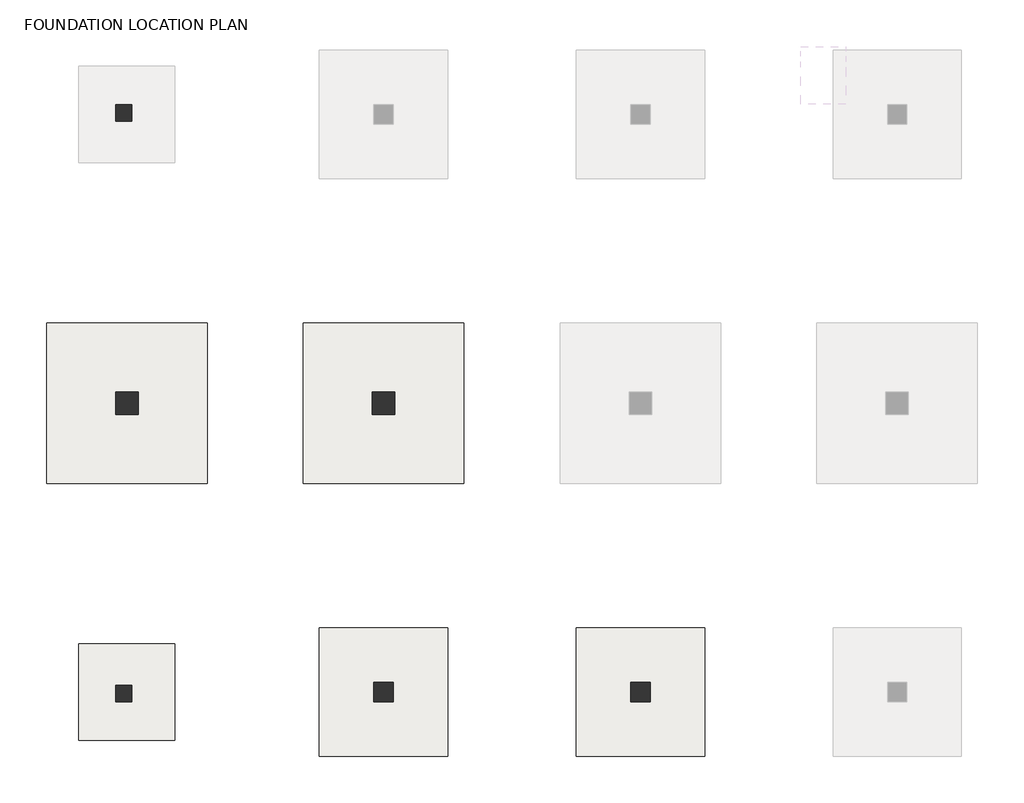
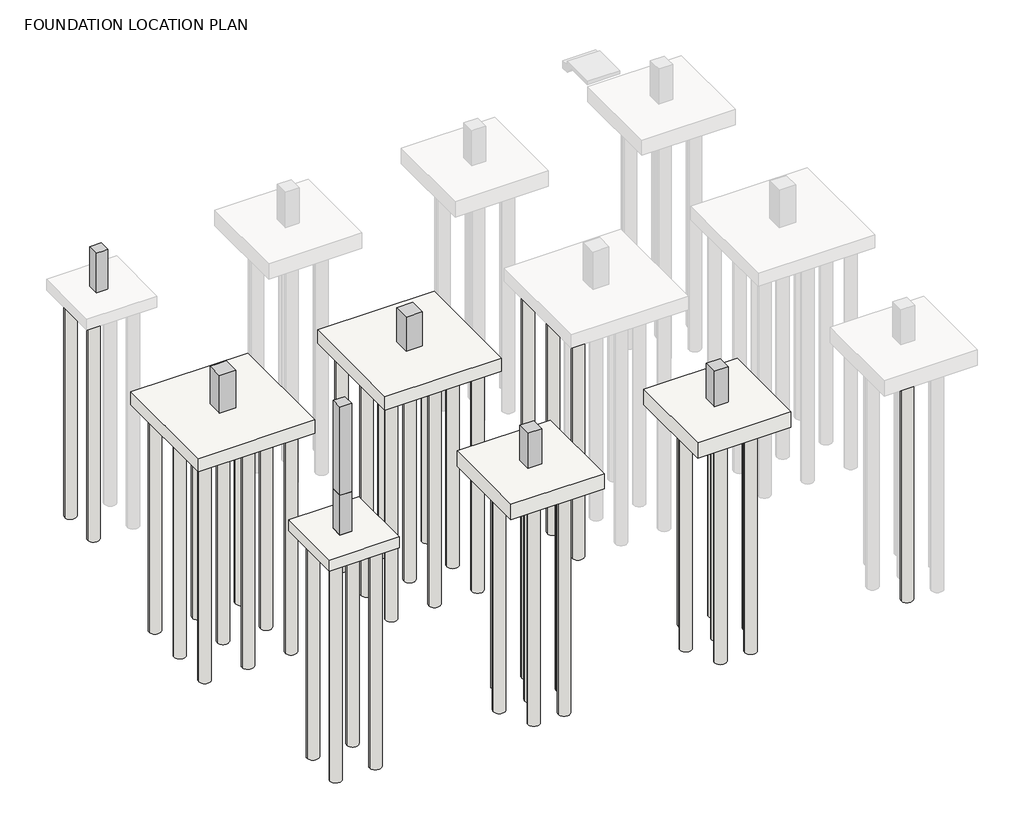
# One storey, part 1 of 3: 47 slabs, 7 columns.
"""IFC4 building model written with IfcOpenShell, lengths in millimetres."""

from ifc_helpers import new_model, si_unit, point, frame, frame_2d, origin, place, context, project, spatial, polyline, circle_curve, trimmed, segment, composite_curve, outline, extrude, faceted_brep, element, save

model = new_model("IFC4")

# Units and contexts
model_context = context("Model", 3, world=origin())
ifc_project = project(units=[si_unit("LENGTHUNIT", "METRE", prefix="MILLI")], contexts=[model_context])

# Site, building, storey
site = spatial("IfcSite", under=ifc_project)
building = spatial("IfcBuilding", under=site)
storey = spatial("IfcBuildingStorey", under=building, Name="FOUNDATION LOCATION PLAN", Elevation=-1699.994759)

# Columns
placement = place(None, origin())
element("IfcColumn", 1, ObjectType="Concrete-Rectangular-Column_R1 : CLS113_RC COLUMN_AG_C1", at=placement, inside=storey, context=model_context, shape_type="Brep", body=[
    faceted_brep([(-350.0, 21199.5208589, -1699.994759), (150.0, 21199.5208589, -1699.994759), (150.0, 20699.5208589, -1699.994759), (-350.0, 20699.5208589, -1699.994759), (150.0, 21199.5208589, -1199.994759), (-350.0, 21199.5208589, -1199.994759), (-350.0, 20699.5208589, -1199.994759), (150.0, 20699.5208589, -1199.994759)], [[[0, 1, 2, 3]], [[4, 5, 6, 7]], [[1, 0, 5, 4]], [[2, 1, 4, 7]], [[3, 2, 7, 6]], [[0, 3, 6, 5]]]),
    faceted_brep([(-350.0, 21199.5208589, 4600.005241), (150.0, 21199.5208589, 4600.005241), (150.0, 21199.5208589, 600.005241), (-99.0, 21199.5208589, 600.005241), (-350.0, 21199.5208589, 600.005241), (-350.0, 21199.5208589, 3950.005241), (-350.0, 21199.5208589, 4550.005241), (150.0, 20699.5208589, 4600.005241), (150.0, 20699.5208589, 4550.005241), (150.0, 20699.5208589, 3950.005241), (150.0, 20699.5208589, 600.005241), (150.0, 20950.5208589, 600.005241), (-350.0, 20699.5208589, 4600.005241), (-350.0, 20699.5208589, 4550.005241), (-350.0, 20699.5208589, 3950.005241), (-350.0, 20699.5208589, 600.005241)], [[[0, 1, 2, 3, 4, 5, 6]], [[1, 7, 8, 9, 10, 11, 2]], [[7, 12, 13, 14, 15, 10, 9, 8]], [[12, 0, 6, 5, 4, 15, 14, 13]], [[1, 0, 12, 7]], [[4, 3, 2, 11, 10, 15]]]),
])
element("IfcColumn", 2, ObjectType="Concrete-Rectangular-Column_R1 : CLS111_RC COLUMN_UG_C1", at=placement, inside=storey, context=model_context, shape_type="Brep", body=[
    faceted_brep([(-350.0, 21199.5208589, -1199.994759), (150.0, 21199.5208589, -1199.994759), (150.0, 20699.5208589, -1199.994759), (-350.0, 20699.5208589, -1199.994759), (-350.0, 21199.5208589, 450.005241), (-350.0, 21199.5208589, 600.005241), (150.0, 21199.5208589, 600.005241), (150.0, 21199.5208589, 450.005241), (150.0, 20699.5208589, 600.005241), (150.0, 20699.5208589, 450.005241), (-350.0, 20699.5208589, 600.005241)], [[[0, 1, 2, 3]], [[1, 0, 4, 5, 6, 7]], [[2, 1, 7, 6, 8, 9]], [[3, 2, 9, 8, 10]], [[0, 3, 10, 5, 4]], [[6, 5, 10, 8]]]),
])
element("IfcColumn", 3, ObjectType="Concrete-Rectangular-Column_R1 : CLS111_RC COLUMN_UG_C1", at=placement, inside=storey, context=model_context, shape_type="Brep", body=[
    faceted_brep([(-350.0, 39299.5208589, -1199.994759), (150.0, 39299.5208589, -1199.994759), (150.0, 38799.5208589, -1199.994759), (-350.0, 38799.5208589, -1199.994759), (-350.0, 39299.5208589, 600.005241), (150.0, 39299.5208589, 600.005241), (150.0, 38999.7368538, 600.005241), (150.0, 38799.7368538, 600.005241), (150.0, 38799.5208589, 600.005241), (150.0, 38799.5208589, 450.005241), (0.0, 38799.5208589, 600.005241), (-350.0, 38799.5208589, 600.005241), (-350.0, 38799.7368538, 600.005241)], [[[0, 1, 2, 3]], [[1, 0, 4, 5]], [[2, 1, 5, 6, 7, 8, 9]], [[3, 2, 9, 8, 10, 11]], [[0, 3, 11, 12, 4]], [[5, 4, 12, 11, 10, 8, 7, 6]]]),
])
element("IfcColumn", 4, ObjectType="Concrete-Rectangular-Column_R1 : CLS111_RC COLUMN_UG_C3", at=placement, inside=storey, context=model_context, shape_type="Brep", body=[
    faceted_brep([(-350.0, 30349.5208589, -1099.994759), (350.0, 30349.5208589, -1099.994759), (350.0, 29649.5208589, -1099.994759), (-350.0, 29649.5208589, -1099.994759), (-350.0, 30349.5208589, 600.005241), (0.0, 30349.5208589, 600.005241), (350.0, 30349.5208589, 600.005241), (350.0, 30349.5208589, 450.005241), (350.0, 29999.5208589, 600.005241), (350.0, 29649.5208589, 600.005241), (-99.0, 29649.5208589, 600.005241), (-350.0, 29649.5208589, 600.005241)], [[[0, 1, 2, 3]], [[1, 0, 4, 5, 6, 7]], [[2, 1, 7, 6, 8, 9]], [[3, 2, 9, 10, 11]], [[0, 3, 11, 4]], [[11, 10, 9, 8, 6, 5, 4]]]),
])
element("IfcColumn", 5, ObjectType="Concrete-Rectangular-Column_R1 : CLS111_RC COLUMN_UG_C3", at=placement, inside=storey, context=model_context, shape_type="SweptSolid", body=[
    extrude(outline(polyline([(7650.0, 30349.5208589), (8350.0, 30349.5208589), (8350.0, 29649.5208589), (7650.0, 29649.5208589), (7650.0, 30349.5208589)])), frame((0.0, 0.0, -1099.994759), z_axis=(0.0, 0.0, 1.0), x_axis=(1.0, 0.0, 0.0)), (0.0, 0.0, 1.0), 1550.0),
])
element("IfcColumn", 6, ObjectType="Concrete-Rectangular-Column_R1 : CLS111_RC COLUMN_UG_C2", at=placement, inside=storey, context=model_context, shape_type="Brep", body=[
    faceted_brep([(7700.0, 21299.5208589, -999.994759), (8300.0, 21299.5208589, -999.994759), (8300.0, 20699.5208589, -999.994759), (7700.0, 20699.5208589, -999.994759), (7700.0, 21299.5208589, 450.005241), (7700.0, 21299.5208589, 600.005241), (8300.0, 21299.5208589, 600.005241), (8300.0, 21299.5208589, 450.005241), (8300.0, 20999.5208589, 600.005241), (8300.0, 20699.5208589, 600.005241), (7700.0, 20699.5208589, 600.005241), (7700.0, 20999.5208589, 600.005241)], [[[0, 1, 2, 3]], [[1, 0, 4, 5, 6, 7]], [[2, 1, 7, 6, 8, 9]], [[3, 2, 9, 10]], [[0, 3, 10, 11, 5, 4]], [[6, 5, 11, 10, 9, 8]]]),
])
element("IfcColumn", 7, ObjectType="Concrete-Rectangular-Column_R1 : CLS111_RC COLUMN_UG_C2", at=placement, inside=storey, context=model_context, shape_type="Brep", body=[
    faceted_brep([(15700.0, 21299.5208589, -999.994759), (16300.0, 21299.5208589, -999.994759), (16300.0, 20699.5208589, -999.994759), (15700.0, 20699.5208589, -999.994759), (15700.0, 21299.5208589, 450.005241), (15700.0, 21299.5208589, 600.005241), (16300.0, 21299.5208589, 600.005241), (16300.0, 21299.5208589, 450.005241), (16300.0, 20999.5208589, 600.005241), (16300.0, 20699.5208589, 600.005241), (15700.0, 20699.5208589, 600.005241), (15700.0, 20999.5208589, 600.005241)], [[[0, 1, 2, 3]], [[1, 0, 4, 5, 6, 7]], [[2, 1, 7, 6, 8, 9]], [[3, 2, 9, 10]], [[0, 3, 10, 11, 5, 4]], [[6, 5, 11, 10, 9, 8]]]),
])

# Slabs
element("IfcSlab", 8, ObjectType="Footing-Rectangular_R1 : FTS301_Footing-Rectangular_3000x3000x500_F1", at=placement, inside=storey, context=model_context, shape_type="SweptSolid", body=[
    extrude(outline(polyline([(1500.0, 22499.5208589), (1500.0, 19499.5208589), (-1500.0, 19499.5208589), (-1500.0, 22499.5208589), (1500.0, 22499.5208589)])), frame((0.0, 0.0, -1699.994759), z_axis=(0.0, 0.0, 1.0), x_axis=(1.0, 0.0, 0.0)), (0.0, 0.0, 1.0), 500.0),
])
element("IfcSlab", 9, ObjectType="Footing-Rectangular_R1 : FTS301_Footing-Rectangular_4000x4000x700_F2", at=placement, inside=storey, context=model_context, shape_type="SweptSolid", body=[
    extrude(outline(polyline([(10000.0, 22999.5208589), (10000.0, 18999.5208589), (6000.0, 18999.5208589), (6000.0, 22999.5208589), (10000.0, 22999.5208589)])), frame((0.0, 0.0, -1699.994759), z_axis=(0.0, 0.0, 1.0), x_axis=(1.0, 0.0, 0.0)), (0.0, 0.0, 1.0), 700.0),
])
element("IfcSlab", 10, ObjectType="Footing-Rectangular_R1 : FTS301_Footing-Rectangular_4000x4000x700_F2", at=placement, inside=storey, context=model_context, shape_type="SweptSolid", body=[
    extrude(outline(polyline([(18000.0, 22999.5208589), (18000.0, 18999.5208589), (14000.0, 18999.5208589), (14000.0, 22999.5208589), (18000.0, 22999.5208589)])), frame((0.0, 0.0, -1699.994759), z_axis=(0.0, 0.0, 1.0), x_axis=(1.0, 0.0, 0.0)), (0.0, 0.0, 1.0), 700.0),
])
element("IfcSlab", 11, ObjectType="Footing-Rectangular_R1 : FTS301_Footing-Rectangular_5000x5000x600_F3", at=placement, inside=storey, context=model_context, shape_type="SweptSolid", body=[
    extrude(outline(polyline([(2500.0, 32499.5208589), (2500.0, 27499.5208589), (-2500.0, 27499.5208589), (-2500.0, 32499.5208589), (2500.0, 32499.5208589)])), frame((0.0, 0.0, -1699.994759), z_axis=(0.0, 0.0, 1.0), x_axis=(1.0, 0.0, 0.0)), (0.0, 0.0, 1.0), 600.0),
])
element("IfcSlab", 12, ObjectType="Footing-Rectangular_R1 : FTS301_Footing-Rectangular_5000x5000x600_F3", at=placement, inside=storey, context=model_context, shape_type="SweptSolid", body=[
    extrude(outline(polyline([(10500.0, 32499.5208589), (10500.0, 27499.5208589), (5500.0, 27499.5208589), (5500.0, 32499.5208589), (10500.0, 32499.5208589)])), frame((0.0, 0.0, -1699.994759), z_axis=(0.0, 0.0, 1.0), x_axis=(1.0, 0.0, 0.0)), (0.0, 0.0, 1.0), 600.0),
])
element("IfcSlab", 13, ObjectType="HEC_PILE : FTPS102_D500", at=placement, inside=storey, context=model_context, shape_type="SweptSolid", body=[
    extrude(outline(composite_curve([segment(trimmed(circle_curve(frame_2d((7350.0, 19649.5208589)), 250.0), [point((7600.0, 19649.5208589))], [point((7100.0, 19649.5208589))], False, "CARTESIAN"), True, "CONTINUOUS"), segment(trimmed(circle_curve(frame_2d((7350.0, 19649.5208589)), 250.0), [point((7100.0, 19649.5208589))], [point((7600.0, 19649.5208589))], False, "CARTESIAN"), True, "CONTINUOUS")], self_intersect=False)), frame((0.0, 0.0, -11749.994759), z_axis=(0.0, 0.0, 1.0), x_axis=(1.0, 0.0, 0.0)), (0.0, 0.0, 1.0), 10150.0),
])
element("IfcSlab", 14, ObjectType="HEC_PILE : FTPS102_D500", at=placement, inside=storey, context=model_context, shape_type="SweptSolid", body=[
    extrude(outline(composite_curve([segment(trimmed(circle_curve(frame_2d((8650.0, 19649.5208589)), 250.0), [point((8400.0, 19649.5208589))], [point((8900.0, 19649.5208589))], False, "CARTESIAN"), True, "CONTINUOUS"), segment(trimmed(circle_curve(frame_2d((8650.0, 19649.5208589)), 250.0), [point((8900.0, 19649.5208589))], [point((8400.0, 19649.5208589))], False, "CARTESIAN"), True, "CONTINUOUS")], self_intersect=False)), frame((0.0, 0.0, -11749.994759), z_axis=(0.0, 0.0, 1.0), x_axis=(1.0, 0.0, 0.0)), (0.0, 0.0, 1.0), 10150.0),
])
element("IfcSlab", 15, ObjectType="HEC_PILE : FTPS102_D500", at=placement, inside=storey, context=model_context, shape_type="SweptSolid", body=[
    extrude(outline(composite_curve([segment(trimmed(circle_curve(frame_2d((6650.0, 20999.5208589)), 250.0), [point((6900.0, 20999.5208589))], [point((6400.0, 20999.5208589))], False, "CARTESIAN"), True, "CONTINUOUS"), segment(trimmed(circle_curve(frame_2d((6650.0, 20999.5208589)), 250.0), [point((6400.0, 20999.5208589))], [point((6900.0, 20999.5208589))], False, "CARTESIAN"), True, "CONTINUOUS")], self_intersect=False)), frame((0.0, 0.0, -11749.994759), z_axis=(0.0, 0.0, 1.0), x_axis=(1.0, 0.0, 0.0)), (0.0, 0.0, 1.0), 10150.0),
])
element("IfcSlab", 16, ObjectType="HEC_PILE : FTPS102_D500", at=placement, inside=storey, context=model_context, shape_type="SweptSolid", body=[
    extrude(outline(composite_curve([segment(trimmed(circle_curve(frame_2d((8000.0, 20999.5208589)), 250.0), [point((8250.0, 20999.5208589))], [point((7750.0, 20999.5208589))], False, "CARTESIAN"), True, "CONTINUOUS"), segment(trimmed(circle_curve(frame_2d((8000.0, 20999.5208589)), 250.0), [point((7750.0, 20999.5208589))], [point((8250.0, 20999.5208589))], False, "CARTESIAN"), True, "CONTINUOUS")], self_intersect=False)), frame((0.0, 0.0, -11749.994759), z_axis=(0.0, 0.0, 1.0), x_axis=(1.0, 0.0, 0.0)), (0.0, 0.0, 1.0), 10150.0),
])
element("IfcSlab", 17, ObjectType="HEC_PILE : FTPS102_D500", at=placement, inside=storey, context=model_context, shape_type="SweptSolid", body=[
    extrude(outline(composite_curve([segment(trimmed(circle_curve(frame_2d((9350.0, 20999.5208589)), 250.0), [point((9100.0, 20999.5208589))], [point((9600.0, 20999.5208589))], False, "CARTESIAN"), True, "CONTINUOUS"), segment(trimmed(circle_curve(frame_2d((9350.0, 20999.5208589)), 250.0), [point((9600.0, 20999.5208589))], [point((9100.0, 20999.5208589))], False, "CARTESIAN"), True, "CONTINUOUS")], self_intersect=False)), frame((0.0, 0.0, -11749.994759), z_axis=(0.0, 0.0, 1.0), x_axis=(1.0, 0.0, 0.0)), (0.0, 0.0, 1.0), 10150.0),
])
element("IfcSlab", 18, ObjectType="HEC_PILE : FTPS102_D500", at=placement, inside=storey, context=model_context, shape_type="SweptSolid", body=[
    extrude(outline(composite_curve([segment(trimmed(circle_curve(frame_2d((7350.0, 22349.5208589)), 250.0), [point((7600.0, 22349.5208589))], [point((7100.0, 22349.5208589))], False, "CARTESIAN"), True, "CONTINUOUS"), segment(trimmed(circle_curve(frame_2d((7350.0, 22349.5208589)), 250.0), [point((7100.0, 22349.5208589))], [point((7600.0, 22349.5208589))], False, "CARTESIAN"), True, "CONTINUOUS")], self_intersect=False)), frame((0.0, 0.0, -11749.994759), z_axis=(0.0, 0.0, 1.0), x_axis=(1.0, 0.0, 0.0)), (0.0, 0.0, 1.0), 10150.0),
])
element("IfcSlab", 19, ObjectType="HEC_PILE : FTPS102_D500", at=placement, inside=storey, context=model_context, shape_type="SweptSolid", body=[
    extrude(outline(composite_curve([segment(trimmed(circle_curve(frame_2d((8650.0, 22349.5208589)), 250.0), [point((8400.0, 22349.5208589))], [point((8900.0, 22349.5208589))], False, "CARTESIAN"), True, "CONTINUOUS"), segment(trimmed(circle_curve(frame_2d((8650.0, 22349.5208589)), 250.0), [point((8900.0, 22349.5208589))], [point((8400.0, 22349.5208589))], False, "CARTESIAN"), True, "CONTINUOUS")], self_intersect=False)), frame((0.0, 0.0, -11749.994759), z_axis=(0.0, 0.0, 1.0), x_axis=(1.0, 0.0, 0.0)), (0.0, 0.0, 1.0), 10150.0),
])
element("IfcSlab", 20, ObjectType="HEC_PILE : FTPS102_D500", at=placement, inside=storey, context=model_context, shape_type="SweptSolid", body=[
    extrude(outline(composite_curve([segment(trimmed(circle_curve(frame_2d((-850.0, 39849.5208589)), 250.0), [point((-600.0, 39849.5208589))], [point((-1100.0, 39849.5208589))], False, "CARTESIAN"), True, "CONTINUOUS"), segment(trimmed(circle_curve(frame_2d((-850.0, 39849.5208589)), 250.0), [point((-1100.0, 39849.5208589))], [point((-600.0, 39849.5208589))], False, "CARTESIAN"), True, "CONTINUOUS")], self_intersect=False)), frame((0.0, 0.0, -11749.994759), z_axis=(0.0, 0.0, 1.0), x_axis=(1.0, 0.0, 0.0)), (0.0, 0.0, 1.0), 10150.0),
])
element("IfcSlab", 21, ObjectType="HEC_PILE : FTPS102_D500", at=placement, inside=storey, context=model_context, shape_type="SweptSolid", body=[
    extrude(outline(composite_curve([segment(trimmed(circle_curve(frame_2d((-850.0, 21849.5208589)), 250.0), [point((-600.0, 21849.5208589))], [point((-1100.0, 21849.5208589))], False, "CARTESIAN"), True, "CONTINUOUS"), segment(trimmed(circle_curve(frame_2d((-850.0, 21849.5208589)), 250.0), [point((-1100.0, 21849.5208589))], [point((-600.0, 21849.5208589))], False, "CARTESIAN"), True, "CONTINUOUS")], self_intersect=False)), frame((0.0, 0.0, -11749.994759), z_axis=(0.0, 0.0, 1.0), x_axis=(1.0, 0.0, 0.0)), (0.0, 0.0, 1.0), 10150.0),
])
element("IfcSlab", 22, ObjectType="HEC_PILE : FTPS102_D500", at=placement, inside=storey, context=model_context, shape_type="SweptSolid", body=[
    extrude(outline(composite_curve([segment(trimmed(circle_curve(frame_2d((850.0, 21849.5208589)), 250.0), [point((600.0, 21849.5208589))], [point((1100.0, 21849.5208589))], False, "CARTESIAN"), True, "CONTINUOUS"), segment(trimmed(circle_curve(frame_2d((850.0, 21849.5208589)), 250.0), [point((1100.0, 21849.5208589))], [point((600.0, 21849.5208589))], False, "CARTESIAN"), True, "CONTINUOUS")], self_intersect=False)), frame((0.0, 0.0, -11749.994759), z_axis=(0.0, 0.0, 1.0), x_axis=(1.0, 0.0, 0.0)), (0.0, 0.0, 1.0), 10150.0),
])
element("IfcSlab", 23, ObjectType="HEC_PILE : FTPS102_D500", at=placement, inside=storey, context=model_context, shape_type="SweptSolid", body=[
    extrude(outline(composite_curve([segment(trimmed(circle_curve(frame_2d((-850.0, 20149.5208589)), 250.0), [point((-600.0, 20149.5208589))], [point((-1100.0, 20149.5208589))], False, "CARTESIAN"), True, "CONTINUOUS"), segment(trimmed(circle_curve(frame_2d((-850.0, 20149.5208589)), 250.0), [point((-1100.0, 20149.5208589))], [point((-600.0, 20149.5208589))], False, "CARTESIAN"), True, "CONTINUOUS")], self_intersect=False)), frame((0.0, 0.0, -11749.994759), z_axis=(0.0, 0.0, 1.0), x_axis=(1.0, 0.0, 0.0)), (0.0, 0.0, 1.0), 10150.0),
])
element("IfcSlab", 24, ObjectType="HEC_PILE : FTPS102_D500", at=placement, inside=storey, context=model_context, shape_type="SweptSolid", body=[
    extrude(outline(composite_curve([segment(trimmed(circle_curve(frame_2d((850.0, 20149.5208589)), 250.0), [point((600.0, 20149.5208589))], [point((1100.0, 20149.5208589))], False, "CARTESIAN"), True, "CONTINUOUS"), segment(trimmed(circle_curve(frame_2d((850.0, 20149.5208589)), 250.0), [point((1100.0, 20149.5208589))], [point((600.0, 20149.5208589))], False, "CARTESIAN"), True, "CONTINUOUS")], self_intersect=False)), frame((0.0, 0.0, -11749.994759), z_axis=(0.0, 0.0, 1.0), x_axis=(1.0, 0.0, 0.0)), (0.0, 0.0, 1.0), 10150.0),
])
element("IfcSlab", 25, ObjectType="HEC_PILE : FTPS102_D500", at=placement, inside=storey, context=model_context, shape_type="SweptSolid", body=[
    extrude(outline(composite_curve([segment(trimmed(circle_curve(frame_2d((15350.0, 19649.5208589)), 250.0), [point((15600.0, 19649.5208589))], [point((15100.0, 19649.5208589))], False, "CARTESIAN"), True, "CONTINUOUS"), segment(trimmed(circle_curve(frame_2d((15350.0, 19649.5208589)), 250.0), [point((15100.0, 19649.5208589))], [point((15600.0, 19649.5208589))], False, "CARTESIAN"), True, "CONTINUOUS")], self_intersect=False)), frame((0.0, 0.0, -11749.994759), z_axis=(0.0, 0.0, 1.0), x_axis=(1.0, 0.0, 0.0)), (0.0, 0.0, 1.0), 10150.0),
])
element("IfcSlab", 26, ObjectType="HEC_PILE : FTPS102_D500", at=placement, inside=storey, context=model_context, shape_type="SweptSolid", body=[
    extrude(outline(composite_curve([segment(trimmed(circle_curve(frame_2d((16650.0, 19649.5208589)), 250.0), [point((16400.0, 19649.5208589))], [point((16900.0, 19649.5208589))], False, "CARTESIAN"), True, "CONTINUOUS"), segment(trimmed(circle_curve(frame_2d((16650.0, 19649.5208589)), 250.0), [point((16900.0, 19649.5208589))], [point((16400.0, 19649.5208589))], False, "CARTESIAN"), True, "CONTINUOUS")], self_intersect=False)), frame((0.0, 0.0, -11749.994759), z_axis=(0.0, 0.0, 1.0), x_axis=(1.0, 0.0, 0.0)), (0.0, 0.0, 1.0), 10150.0),
])
element("IfcSlab", 27, ObjectType="HEC_PILE : FTPS102_D500", at=placement, inside=storey, context=model_context, shape_type="SweptSolid", body=[
    extrude(outline(composite_curve([segment(trimmed(circle_curve(frame_2d((14650.0, 20999.5208589)), 250.0), [point((14900.0, 20999.5208589))], [point((14400.0, 20999.5208589))], False, "CARTESIAN"), True, "CONTINUOUS"), segment(trimmed(circle_curve(frame_2d((14650.0, 20999.5208589)), 250.0), [point((14400.0, 20999.5208589))], [point((14900.0, 20999.5208589))], False, "CARTESIAN"), True, "CONTINUOUS")], self_intersect=False)), frame((0.0, 0.0, -11749.994759), z_axis=(0.0, 0.0, 1.0), x_axis=(1.0, 0.0, 0.0)), (0.0, 0.0, 1.0), 10150.0),
])
element("IfcSlab", 28, ObjectType="HEC_PILE : FTPS102_D500", at=placement, inside=storey, context=model_context, shape_type="SweptSolid", body=[
    extrude(outline(composite_curve([segment(trimmed(circle_curve(frame_2d((16000.0, 20999.5208589)), 250.0), [point((16250.0, 20999.5208589))], [point((15750.0, 20999.5208589))], False, "CARTESIAN"), True, "CONTINUOUS"), segment(trimmed(circle_curve(frame_2d((16000.0, 20999.5208589)), 250.0), [point((15750.0, 20999.5208589))], [point((16250.0, 20999.5208589))], False, "CARTESIAN"), True, "CONTINUOUS")], self_intersect=False)), frame((0.0, 0.0, -11749.994759), z_axis=(0.0, 0.0, 1.0), x_axis=(1.0, 0.0, 0.0)), (0.0, 0.0, 1.0), 10150.0),
])
element("IfcSlab", 29, ObjectType="HEC_PILE : FTPS102_D500", at=placement, inside=storey, context=model_context, shape_type="SweptSolid", body=[
    extrude(outline(composite_curve([segment(trimmed(circle_curve(frame_2d((17350.0, 20999.5208589)), 250.0), [point((17100.0, 20999.5208589))], [point((17600.0, 20999.5208589))], False, "CARTESIAN"), True, "CONTINUOUS"), segment(trimmed(circle_curve(frame_2d((17350.0, 20999.5208589)), 250.0), [point((17600.0, 20999.5208589))], [point((17100.0, 20999.5208589))], False, "CARTESIAN"), True, "CONTINUOUS")], self_intersect=False)), frame((0.0, 0.0, -11749.994759), z_axis=(0.0, 0.0, 1.0), x_axis=(1.0, 0.0, 0.0)), (0.0, 0.0, 1.0), 10150.0),
])
element("IfcSlab", 30, ObjectType="HEC_PILE : FTPS102_D500", at=placement, inside=storey, context=model_context, shape_type="SweptSolid", body=[
    extrude(outline(composite_curve([segment(trimmed(circle_curve(frame_2d((15350.0, 22349.5208589)), 250.0), [point((15600.0, 22349.5208589))], [point((15100.0, 22349.5208589))], False, "CARTESIAN"), True, "CONTINUOUS"), segment(trimmed(circle_curve(frame_2d((15350.0, 22349.5208589)), 250.0), [point((15100.0, 22349.5208589))], [point((15600.0, 22349.5208589))], False, "CARTESIAN"), True, "CONTINUOUS")], self_intersect=False)), frame((0.0, 0.0, -11749.994759), z_axis=(0.0, 0.0, 1.0), x_axis=(1.0, 0.0, 0.0)), (0.0, 0.0, 1.0), 10150.0),
])
element("IfcSlab", 31, ObjectType="HEC_PILE : FTPS102_D500", at=placement, inside=storey, context=model_context, shape_type="SweptSolid", body=[
    extrude(outline(composite_curve([segment(trimmed(circle_curve(frame_2d((16650.0, 22349.5208589)), 250.0), [point((16400.0, 22349.5208589))], [point((16900.0, 22349.5208589))], False, "CARTESIAN"), True, "CONTINUOUS"), segment(trimmed(circle_curve(frame_2d((16650.0, 22349.5208589)), 250.0), [point((16900.0, 22349.5208589))], [point((16400.0, 22349.5208589))], False, "CARTESIAN"), True, "CONTINUOUS")], self_intersect=False)), frame((0.0, 0.0, -11749.994759), z_axis=(0.0, 0.0, 1.0), x_axis=(1.0, 0.0, 0.0)), (0.0, 0.0, 1.0), 10150.0),
])
element("IfcSlab", 32, ObjectType="HEC_PILE : FTPS102_D500", at=placement, inside=storey, context=model_context, shape_type="SweptSolid", body=[
    extrude(outline(composite_curve([segment(trimmed(circle_curve(frame_2d((23350.0, 19649.5208589)), 250.0), [point((23600.0, 19649.5208589))], [point((23100.0, 19649.5208589))], False, "CARTESIAN"), True, "CONTINUOUS"), segment(trimmed(circle_curve(frame_2d((23350.0, 19649.5208589)), 250.0), [point((23100.0, 19649.5208589))], [point((23600.0, 19649.5208589))], False, "CARTESIAN"), True, "CONTINUOUS")], self_intersect=False)), frame((0.0, 0.0, -11749.994759), z_axis=(0.0, 0.0, 1.0), x_axis=(1.0, 0.0, 0.0)), (0.0, 0.0, 1.0), 10150.0),
])
element("IfcSlab", 33, ObjectType="HEC_PILE : FTPS102_D500", at=placement, inside=storey, context=model_context, shape_type="SweptSolid", body=[
    extrude(outline(composite_curve([segment(trimmed(circle_curve(frame_2d((-1850.0, 29999.5208589)), 250.0), [point((-1600.0, 29999.5208589))], [point((-2100.0, 29999.5208589))], False, "CARTESIAN"), True, "CONTINUOUS"), segment(trimmed(circle_curve(frame_2d((-1850.0, 29999.5208589)), 250.0), [point((-2100.0, 29999.5208589))], [point((-1600.0, 29999.5208589))], False, "CARTESIAN"), True, "CONTINUOUS")], self_intersect=False)), frame((0.0, 0.0, -11749.994759), z_axis=(0.0, 0.0, 1.0), x_axis=(1.0, 0.0, 0.0)), (0.0, 0.0, 1.0), 10150.0),
])
element("IfcSlab", 34, ObjectType="HEC_PILE : FTPS102_D500", at=placement, inside=storey, context=model_context, shape_type="SweptSolid", body=[
    extrude(outline(composite_curve([segment(trimmed(circle_curve(frame_2d((1850.0, 29999.5208589)), 250.0), [point((1600.0, 29999.5208589))], [point((2100.0, 29999.5208589))], False, "CARTESIAN"), True, "CONTINUOUS"), segment(trimmed(circle_curve(frame_2d((1850.0, 29999.5208589)), 250.0), [point((2100.0, 29999.5208589))], [point((1600.0, 29999.5208589))], False, "CARTESIAN"), True, "CONTINUOUS")], self_intersect=False)), frame((0.0, 0.0, -11749.994759), z_axis=(0.0, 0.0, 1.0), x_axis=(1.0, 0.0, 0.0)), (0.0, 0.0, 1.0), 10150.0),
])
element("IfcSlab", 35, ObjectType="HEC_PILE : FTPS102_D500", at=placement, inside=storey, context=model_context, shape_type="SweptSolid", body=[
    extrude(outline(composite_curve([segment(trimmed(circle_curve(frame_2d((0.0, 29999.5208589)), 250.0), [point((-250.0, 29999.5208589))], [point((250.0, 29999.5208589))], False, "CARTESIAN"), True, "CONTINUOUS"), segment(trimmed(circle_curve(frame_2d((0.0, 29999.5208589)), 250.0), [point((250.0, 29999.5208589))], [point((-250.0, 29999.5208589))], False, "CARTESIAN"), True, "CONTINUOUS")], self_intersect=False)), frame((0.0, 0.0, -11749.994759), z_axis=(0.0, 0.0, 1.0), x_axis=(1.0, 0.0, 0.0)), (0.0, 0.0, 1.0), 10150.0),
])
element("IfcSlab", 36, ObjectType="HEC_PILE : FTPS102_D500", at=placement, inside=storey, context=model_context, shape_type="SweptSolid", body=[
    extrude(outline(composite_curve([segment(trimmed(circle_curve(frame_2d((-1850.0, 31849.5208589)), 250.0), [point((-1600.0, 31849.5208589))], [point((-2100.0, 31849.5208589))], False, "CARTESIAN"), True, "CONTINUOUS"), segment(trimmed(circle_curve(frame_2d((-1850.0, 31849.5208589)), 250.0), [point((-2100.0, 31849.5208589))], [point((-1600.0, 31849.5208589))], False, "CARTESIAN"), True, "CONTINUOUS")], self_intersect=False)), frame((0.0, 0.0, -11749.994759), z_axis=(0.0, 0.0, 1.0), x_axis=(1.0, 0.0, 0.0)), (0.0, 0.0, 1.0), 10150.0),
])
element("IfcSlab", 37, ObjectType="HEC_PILE : FTPS102_D500", at=placement, inside=storey, context=model_context, shape_type="SweptSolid", body=[
    extrude(outline(composite_curve([segment(trimmed(circle_curve(frame_2d((1850.0, 31849.5208589)), 250.0), [point((1600.0, 31849.5208589))], [point((2100.0, 31849.5208589))], False, "CARTESIAN"), True, "CONTINUOUS"), segment(trimmed(circle_curve(frame_2d((1850.0, 31849.5208589)), 250.0), [point((2100.0, 31849.5208589))], [point((1600.0, 31849.5208589))], False, "CARTESIAN"), True, "CONTINUOUS")], self_intersect=False)), frame((0.0, 0.0, -11749.994759), z_axis=(0.0, 0.0, 1.0), x_axis=(1.0, 0.0, 0.0)), (0.0, 0.0, 1.0), 10150.0),
])
element("IfcSlab", 38, ObjectType="HEC_PILE : FTPS102_D500", at=placement, inside=storey, context=model_context, shape_type="SweptSolid", body=[
    extrude(outline(composite_curve([segment(trimmed(circle_curve(frame_2d((0.0, 31849.5208589)), 250.0), [point((-250.0, 31849.5208589))], [point((250.0, 31849.5208589))], False, "CARTESIAN"), True, "CONTINUOUS"), segment(trimmed(circle_curve(frame_2d((0.0, 31849.5208589)), 250.0), [point((250.0, 31849.5208589))], [point((-250.0, 31849.5208589))], False, "CARTESIAN"), True, "CONTINUOUS")], self_intersect=False)), frame((0.0, 0.0, -11749.994759), z_axis=(0.0, 0.0, 1.0), x_axis=(1.0, 0.0, 0.0)), (0.0, 0.0, 1.0), 10150.0),
])
element("IfcSlab", 39, ObjectType="HEC_PILE : FTPS102_D500", at=placement, inside=storey, context=model_context, shape_type="SweptSolid", body=[
    extrude(outline(composite_curve([segment(trimmed(circle_curve(frame_2d((-1850.0, 28149.5208589)), 250.0), [point((-1600.0, 28149.5208589))], [point((-2100.0, 28149.5208589))], False, "CARTESIAN"), True, "CONTINUOUS"), segment(trimmed(circle_curve(frame_2d((-1850.0, 28149.5208589)), 250.0), [point((-2100.0, 28149.5208589))], [point((-1600.0, 28149.5208589))], False, "CARTESIAN"), True, "CONTINUOUS")], self_intersect=False)), frame((0.0, 0.0, -11749.994759), z_axis=(0.0, 0.0, 1.0), x_axis=(1.0, 0.0, 0.0)), (0.0, 0.0, 1.0), 10150.0),
])
element("IfcSlab", 40, ObjectType="HEC_PILE : FTPS102_D500", at=placement, inside=storey, context=model_context, shape_type="SweptSolid", body=[
    extrude(outline(composite_curve([segment(trimmed(circle_curve(frame_2d((1850.0, 28149.5208589)), 250.0), [point((1600.0, 28149.5208589))], [point((2100.0, 28149.5208589))], False, "CARTESIAN"), True, "CONTINUOUS"), segment(trimmed(circle_curve(frame_2d((1850.0, 28149.5208589)), 250.0), [point((2100.0, 28149.5208589))], [point((1600.0, 28149.5208589))], False, "CARTESIAN"), True, "CONTINUOUS")], self_intersect=False)), frame((0.0, 0.0, -11749.994759), z_axis=(0.0, 0.0, 1.0), x_axis=(1.0, 0.0, 0.0)), (0.0, 0.0, 1.0), 10150.0),
])
element("IfcSlab", 41, ObjectType="HEC_PILE : FTPS102_D500", at=placement, inside=storey, context=model_context, shape_type="SweptSolid", body=[
    extrude(outline(composite_curve([segment(trimmed(circle_curve(frame_2d((0.0, 28149.5208589)), 250.0), [point((-250.0, 28149.5208589))], [point((250.0, 28149.5208589))], False, "CARTESIAN"), True, "CONTINUOUS"), segment(trimmed(circle_curve(frame_2d((0.0, 28149.5208589)), 250.0), [point((250.0, 28149.5208589))], [point((-250.0, 28149.5208589))], False, "CARTESIAN"), True, "CONTINUOUS")], self_intersect=False)), frame((0.0, 0.0, -11749.994759), z_axis=(0.0, 0.0, 1.0), x_axis=(1.0, 0.0, 0.0)), (0.0, 0.0, 1.0), 10150.0),
])
element("IfcSlab", 42, ObjectType="HEC_PILE : FTPS102_D500", at=placement, inside=storey, context=model_context, shape_type="SweptSolid", body=[
    extrude(outline(composite_curve([segment(trimmed(circle_curve(frame_2d((6150.0, 29999.5208589)), 250.0), [point((6400.0, 29999.5208589))], [point((5900.0, 29999.5208589))], False, "CARTESIAN"), True, "CONTINUOUS"), segment(trimmed(circle_curve(frame_2d((6150.0, 29999.5208589)), 250.0), [point((5900.0, 29999.5208589))], [point((6400.0, 29999.5208589))], False, "CARTESIAN"), True, "CONTINUOUS")], self_intersect=False)), frame((0.0, 0.0, -11749.994759), z_axis=(0.0, 0.0, 1.0), x_axis=(1.0, 0.0, 0.0)), (0.0, 0.0, 1.0), 10150.0),
])
element("IfcSlab", 43, ObjectType="HEC_PILE : FTPS102_D500", at=placement, inside=storey, context=model_context, shape_type="SweptSolid", body=[
    extrude(outline(composite_curve([segment(trimmed(circle_curve(frame_2d((9850.0, 29999.5208589)), 250.0), [point((9600.0, 29999.5208589))], [point((10100.0, 29999.5208589))], False, "CARTESIAN"), True, "CONTINUOUS"), segment(trimmed(circle_curve(frame_2d((9850.0, 29999.5208589)), 250.0), [point((10100.0, 29999.5208589))], [point((9600.0, 29999.5208589))], False, "CARTESIAN"), True, "CONTINUOUS")], self_intersect=False)), frame((0.0, 0.0, -11749.994759), z_axis=(0.0, 0.0, 1.0), x_axis=(1.0, 0.0, 0.0)), (0.0, 0.0, 1.0), 10150.0),
])
element("IfcSlab", 44, ObjectType="HEC_PILE : FTPS102_D500", at=placement, inside=storey, context=model_context, shape_type="SweptSolid", body=[
    extrude(outline(composite_curve([segment(trimmed(circle_curve(frame_2d((8000.0, 29999.5208589)), 250.0), [point((7750.0, 29999.5208589))], [point((8250.0, 29999.5208589))], False, "CARTESIAN"), True, "CONTINUOUS"), segment(trimmed(circle_curve(frame_2d((8000.0, 29999.5208589)), 250.0), [point((8250.0, 29999.5208589))], [point((7750.0, 29999.5208589))], False, "CARTESIAN"), True, "CONTINUOUS")], self_intersect=False)), frame((0.0, 0.0, -11749.994759), z_axis=(0.0, 0.0, 1.0), x_axis=(1.0, 0.0, 0.0)), (0.0, 0.0, 1.0), 10150.0),
])
element("IfcSlab", 45, ObjectType="HEC_PILE : FTPS102_D500", at=placement, inside=storey, context=model_context, shape_type="SweptSolid", body=[
    extrude(outline(composite_curve([segment(trimmed(circle_curve(frame_2d((6150.0, 31849.5208589)), 250.0), [point((6400.0, 31849.5208589))], [point((5900.0, 31849.5208589))], False, "CARTESIAN"), True, "CONTINUOUS"), segment(trimmed(circle_curve(frame_2d((6150.0, 31849.5208589)), 250.0), [point((5900.0, 31849.5208589))], [point((6400.0, 31849.5208589))], False, "CARTESIAN"), True, "CONTINUOUS")], self_intersect=False)), frame((0.0, 0.0, -11749.994759), z_axis=(0.0, 0.0, 1.0), x_axis=(1.0, 0.0, 0.0)), (0.0, 0.0, 1.0), 10150.0),
])
element("IfcSlab", 46, ObjectType="HEC_PILE : FTPS102_D500", at=placement, inside=storey, context=model_context, shape_type="SweptSolid", body=[
    extrude(outline(composite_curve([segment(trimmed(circle_curve(frame_2d((9850.0, 31849.5208589)), 250.0), [point((9600.0, 31849.5208589))], [point((10100.0, 31849.5208589))], False, "CARTESIAN"), True, "CONTINUOUS"), segment(trimmed(circle_curve(frame_2d((9850.0, 31849.5208589)), 250.0), [point((10100.0, 31849.5208589))], [point((9600.0, 31849.5208589))], False, "CARTESIAN"), True, "CONTINUOUS")], self_intersect=False)), frame((0.0, 0.0, -11749.994759), z_axis=(0.0, 0.0, 1.0), x_axis=(1.0, 0.0, 0.0)), (0.0, 0.0, 1.0), 10150.0),
])
element("IfcSlab", 47, ObjectType="HEC_PILE : FTPS102_D500", at=placement, inside=storey, context=model_context, shape_type="SweptSolid", body=[
    extrude(outline(composite_curve([segment(trimmed(circle_curve(frame_2d((8000.0, 31849.5208589)), 250.0), [point((7750.0, 31849.5208589))], [point((8250.0, 31849.5208589))], False, "CARTESIAN"), True, "CONTINUOUS"), segment(trimmed(circle_curve(frame_2d((8000.0, 31849.5208589)), 250.0), [point((8250.0, 31849.5208589))], [point((7750.0, 31849.5208589))], False, "CARTESIAN"), True, "CONTINUOUS")], self_intersect=False)), frame((0.0, 0.0, -11749.994759), z_axis=(0.0, 0.0, 1.0), x_axis=(1.0, 0.0, 0.0)), (0.0, 0.0, 1.0), 10150.0),
])
element("IfcSlab", 48, ObjectType="HEC_PILE : FTPS102_D500", at=placement, inside=storey, context=model_context, shape_type="SweptSolid", body=[
    extrude(outline(composite_curve([segment(trimmed(circle_curve(frame_2d((6150.0, 28149.5208589)), 250.0), [point((6400.0, 28149.5208589))], [point((5900.0, 28149.5208589))], False, "CARTESIAN"), True, "CONTINUOUS"), segment(trimmed(circle_curve(frame_2d((6150.0, 28149.5208589)), 250.0), [point((5900.0, 28149.5208589))], [point((6400.0, 28149.5208589))], False, "CARTESIAN"), True, "CONTINUOUS")], self_intersect=False)), frame((0.0, 0.0, -11749.994759), z_axis=(0.0, 0.0, 1.0), x_axis=(1.0, 0.0, 0.0)), (0.0, 0.0, 1.0), 10150.0),
])
element("IfcSlab", 49, ObjectType="HEC_PILE : FTPS102_D500", at=placement, inside=storey, context=model_context, shape_type="SweptSolid", body=[
    extrude(outline(composite_curve([segment(trimmed(circle_curve(frame_2d((9850.0, 28149.5208589)), 250.0), [point((9600.0, 28149.5208589))], [point((10100.0, 28149.5208589))], False, "CARTESIAN"), True, "CONTINUOUS"), segment(trimmed(circle_curve(frame_2d((9850.0, 28149.5208589)), 250.0), [point((10100.0, 28149.5208589))], [point((9600.0, 28149.5208589))], False, "CARTESIAN"), True, "CONTINUOUS")], self_intersect=False)), frame((0.0, 0.0, -11749.994759), z_axis=(0.0, 0.0, 1.0), x_axis=(1.0, 0.0, 0.0)), (0.0, 0.0, 1.0), 10150.0),
])
element("IfcSlab", 50, ObjectType="HEC_PILE : FTPS102_D500", at=placement, inside=storey, context=model_context, shape_type="SweptSolid", body=[
    extrude(outline(composite_curve([segment(trimmed(circle_curve(frame_2d((8000.0, 28149.5208589)), 250.0), [point((7750.0, 28149.5208589))], [point((8250.0, 28149.5208589))], False, "CARTESIAN"), True, "CONTINUOUS"), segment(trimmed(circle_curve(frame_2d((8000.0, 28149.5208589)), 250.0), [point((8250.0, 28149.5208589))], [point((7750.0, 28149.5208589))], False, "CARTESIAN"), True, "CONTINUOUS")], self_intersect=False)), frame((0.0, 0.0, -11749.994759), z_axis=(0.0, 0.0, 1.0), x_axis=(1.0, 0.0, 0.0)), (0.0, 0.0, 1.0), 10150.0),
])
element("IfcSlab", 51, ObjectType="HEC_PILE : FTPS102_D500", at=placement, inside=storey, context=model_context, shape_type="SweptSolid", body=[
    extrude(outline(composite_curve([segment(trimmed(circle_curve(frame_2d((14150.0, 29999.5208589)), 250.0), [point((14400.0, 29999.5208589))], [point((13900.0, 29999.5208589))], False, "CARTESIAN"), True, "CONTINUOUS"), segment(trimmed(circle_curve(frame_2d((14150.0, 29999.5208589)), 250.0), [point((13900.0, 29999.5208589))], [point((14400.0, 29999.5208589))], False, "CARTESIAN"), True, "CONTINUOUS")], self_intersect=False)), frame((0.0, 0.0, -11749.994759), z_axis=(0.0, 0.0, 1.0), x_axis=(1.0, 0.0, 0.0)), (0.0, 0.0, 1.0), 10150.0),
])
element("IfcSlab", 52, ObjectType="HEC_PILE : FTPS102_D500", at=placement, inside=storey, context=model_context, shape_type="SweptSolid", body=[
    extrude(outline(composite_curve([segment(trimmed(circle_curve(frame_2d((14150.0, 31849.5208589)), 250.0), [point((14400.0, 31849.5208589))], [point((13900.0, 31849.5208589))], False, "CARTESIAN"), True, "CONTINUOUS"), segment(trimmed(circle_curve(frame_2d((14150.0, 31849.5208589)), 250.0), [point((13900.0, 31849.5208589))], [point((14400.0, 31849.5208589))], False, "CARTESIAN"), True, "CONTINUOUS")], self_intersect=False)), frame((0.0, 0.0, -11749.994759), z_axis=(0.0, 0.0, 1.0), x_axis=(1.0, 0.0, 0.0)), (0.0, 0.0, 1.0), 10150.0),
])
element("IfcSlab", 53, ObjectType="HEC_PILE : FTPS102_D500", at=placement, inside=storey, context=model_context, shape_type="SweptSolid", body=[
    extrude(outline(composite_curve([segment(trimmed(circle_curve(frame_2d((14150.0, 28149.5208589)), 250.0), [point((14400.0, 28149.5208589))], [point((13900.0, 28149.5208589))], False, "CARTESIAN"), True, "CONTINUOUS"), segment(trimmed(circle_curve(frame_2d((14150.0, 28149.5208589)), 250.0), [point((13900.0, 28149.5208589))], [point((14400.0, 28149.5208589))], False, "CARTESIAN"), True, "CONTINUOUS")], self_intersect=False)), frame((0.0, 0.0, -11749.994759), z_axis=(0.0, 0.0, 1.0), x_axis=(1.0, 0.0, 0.0)), (0.0, 0.0, 1.0), 10150.0),
])
element("IfcSlab", 54, ObjectType="HEC_PILE : FTPS102_D500", at=placement, inside=storey, context=model_context, shape_type="SweptSolid", body=[
    extrude(outline(composite_curve([segment(trimmed(circle_curve(frame_2d((-850.0, 38149.9528486)), 250.0), [point((-600.0, 38149.9528486))], [point((-1100.0, 38149.9528486))], False, "CARTESIAN"), True, "CONTINUOUS"), segment(trimmed(circle_curve(frame_2d((-850.0, 38149.9528486)), 250.0), [point((-1100.0, 38149.9528486))], [point((-600.0, 38149.9528486))], False, "CARTESIAN"), True, "CONTINUOUS")], self_intersect=False)), frame((0.0, 0.0, -11749.994759), z_axis=(0.0, 0.0, 1.0), x_axis=(1.0, 0.0, 0.0)), (0.0, 0.0, 1.0), 10150.0),
])

save(model, "model.ifc")

# Revit data of these elements
# Project information
#   Building Name = "CENTRAL CONTROL BUILDING"
#   Project Status = "Project Status"
#   Client Name = "현대엔지니어링"
#   Project Address = "서울시 종로구 율곡로 75(계동)"
#   Project Name = "Therma Visayas Energy Project"
#   Project Number = "-"
# Grids (mm)
#   "1": line (0, 44999.521) -> (0, 14999.521)
#   "B": line (-6000, 29999.521) -> (48000, 29999.521)
#   "C": line (-6000, 38999.737) -> (48000, 38999.737)
#   "2": line (8000, 44999.521) -> (8000, 14999.521)
#   "3": line (16000, 44999.521) -> (16000, 14999.521)
#   "4": line (24000, 44999.521) -> (24000, 14999.521)
#   "5": line (32000, 44999.521) -> (32000, 14999.521)
#   "6": line (42000, 44999.521) -> (42000, 14999.521)
#   "A": line (-6000, 20999.521) -> (48000, 20999.521)
# Type "Concrete-Rectangular-Column_R1 : CLS113_RC COLUMN_AG_C1"
#   Type Mark = "C1"
#   Description = "AG RC 기둥"
#   Width = 500 mm
#   Length = 500 mm
#   hec_material3 [instance default] = none
#   hec_material2 [instance default] = A03AE056-00001_Bitumen/Bituminous/Asphalt Coating
#   hec_material1 [instance default] = A03AC035-00001_Form Work (3 times in use)_Flat
#   Structural Material [instance default] = A03AC032-00007_Structural Concrete_Type1_25MPa-30Mpa
# Type "Concrete-Rectangular-Column_R1 : CLS111_RC COLUMN_UG_C1"
#   Description = "AG RC 기둥"
#   Width = 500 mm
#   Length = 500 mm
#   hec_material3 [instance default] = none
#   hec_material2 [instance default] = A03AE056-00001_Bitumen/Bituminous/Asphalt Coating
#   hec_material1 [instance default] = A03AC035-00001_Form Work (3 times in use)_Flat
#   Structural Material [instance default] = A03AC032-00007_Structural Concrete_Type1_25MPa-30Mpa
# Type "Concrete-Rectangular-Column_R1 : CLS111_RC COLUMN_UG_C3"
#   Description = "AG RC 기둥"
#   Width = 700 mm
#   Length = 700 mm
#   hec_material3 [instance default] = none
#   hec_material2 [instance default] = A03AE056-00001_Bitumen/Bituminous/Asphalt Coating
#   hec_material1 [instance default] = A03AC035-00001_Form Work (3 times in use)_Flat
#   Structural Material [instance default] = A03AC032-00007_Structural Concrete_Type1_25MPa-30Mpa
# Type "Concrete-Rectangular-Column_R1 : CLS111_RC COLUMN_UG_C2"
#   Description = "AG RC 기둥"
#   Width = 600 mm
#   Length = 600 mm
#   hec_material3 [instance default] = none
#   hec_material2 [instance default] = A03AE056-00001_Bitumen/Bituminous/Asphalt Coating
#   hec_material1 [instance default] = A03AC035-00001_Form Work (3 times in use)_Flat
#   Structural Material [instance default] = A03AC032-00007_Structural Concrete_Type1_25MPa-30Mpa
# Type "Footing-Rectangular_R1 : FTS301_Footing-Rectangular_3000x3000x500_F1"
#   Type Mark = "F1"
#   Top bar = "D25@300"
#   Description = "UG Shallow Foundation"
#   Bottom bar = "D20@300"
#   Width = 3000 mm
#   Length = 3000 mm
#   Foundation Thickness = 500 mm
#   Structural Material [instance default] = A03AC032-00007_Structural Concrete_Type1_25MPa-30Mpa
#   Assembly Code = ""
# Type "Footing-Rectangular_R1 : FTS301_Footing-Rectangular_4000x4000x700_F2"
#   Type Mark = "F2"
#   Top bar = "D25@300"
#   Description = "UG Shallow Foundation"
#   Bottom bar = "D20@300"
#   Width = 4000 mm
#   Length = 4000 mm
#   Foundation Thickness = 700 mm
#   Structural Material [instance default] = A03AC032-00007_Structural Concrete_Type1_25MPa-30Mpa
#   Assembly Code = ""
# Type "Footing-Rectangular_R1 : FTS301_Footing-Rectangular_5000x5000x600_F3"
#   Type Mark = "F3"
#   Top bar = "D25@300"
#   Description = "UG Shallow Foundation"
#   Bottom bar = "D20@300"
#   Width = 5000 mm
#   Length = 5000 mm
#   Foundation Thickness = 600 mm
#   Structural Material [instance default] = A03AC032-00007_Structural Concrete_Type1_25MPa-30Mpa
#   Assembly Code = ""
# Type "HEC_PILE : FTPS102_D500"
#   Assembly Code = "A1020130"
#   반지름 = 250 mm
#   최소 내포 = 150 mm
#   Diameter = 500 mm
#   Depth = 10000 mm
#   구조 재료 = A02AA014-00001_Piling Work_Reinforced Concrete Pile(Round Type)_Direct Driving
# Element 1 (IfcColumn, "Concrete-Rectangular-Column_R1 : CLS113_RC COLUMN_AG_C1")
#   Mark = "C1"
#   Structural Material = A03AD032-00007_Structural Concrete_25MPa-30MPa
#   hec_material3 = none
#   hec_material2 = A03AE056-00001_Bitumen/Bituminous/Asphalt Coating
#   hec_material1 = A03AC035-00001_Form Work (3 times in use)_Flat
#   Phase Created = New Construction
#   Materials on its faces: "A03AD032-00007_Structural Concrete_25MPa-30MPa"
# Elements 2, 3 (IfcColumn, "Concrete-Rectangular-Column_R1 : CLS111_RC COLUMN_UG_C1")
#   Mark = "C1"
#   Structural Material = A03AC032-00007_Structural Concrete_Type1_25MPa-30Mpa
#   hec_material3 = none
#   hec_material2 = A03AE056-00001_Bitumen/Bituminous/Asphalt Coating
#   hec_material1 = A03AC035-00001_Form Work (3 times in use)_Flat
#   Phase Created = New Construction
#   Materials on its faces: "A03AC032-00007_Structural Concrete_Type1_25MPa-30Mpa"
# Elements 4, 5 (IfcColumn, "Concrete-Rectangular-Column_R1 : CLS111_RC COLUMN_UG_C3")
#   Mark = "C3"
#   Structural Material = A03AC032-00007_Structural Concrete_Type1_25MPa-30Mpa
#   hec_material3 = none
#   hec_material2 = A03AE056-00001_Bitumen/Bituminous/Asphalt Coating
#   hec_material1 = A03AC035-00001_Form Work (3 times in use)_Flat
#   Phase Created = New Construction
#   Materials on its faces: "A03AC032-00007_Structural Concrete_Type1_25MPa-30Mpa"
# Elements 6, 7 (IfcColumn, "Concrete-Rectangular-Column_R1 : CLS111_RC COLUMN_UG_C2")
#   Mark = "C2"
#   Structural Material = A03AC032-00007_Structural Concrete_Type1_25MPa-30Mpa
#   hec_material3 = none
#   hec_material2 = A03AE056-00001_Bitumen/Bituminous/Asphalt Coating
#   hec_material1 = A03AC035-00001_Form Work (3 times in use)_Flat
#   Phase Created = New Construction
#   Materials on its faces: "A03AC032-00007_Structural Concrete_Type1_25MPa-30Mpa"
# Element 8 (IfcSlab, "Footing-Rectangular_R1 : FTS301_Footing-Rectangular_3000x3000x500_F1")
#   Comments = ""
#   Structural Material = A03AC032-00007_Structural Concrete_Type1_25MPa-30Mpa
#   Phase Created = New Construction
#   Materials on its faces: "A03AC032-00007_Structural Concrete_Type1_25MPa-30Mpa"
# Elements 9, 10 (IfcSlab, "Footing-Rectangular_R1 : FTS301_Footing-Rectangular_4000x4000x700_F2")
#   Comments = ""
#   Structural Material = A03AC032-00007_Structural Concrete_Type1_25MPa-30Mpa
#   Phase Created = New Construction
#   Materials on its faces: "A03AC032-00007_Structural Concrete_Type1_25MPa-30Mpa"
# Elements 11, 12 (IfcSlab, "Footing-Rectangular_R1 : FTS301_Footing-Rectangular_5000x5000x600_F3")
#   Comments = ""
#   Structural Material = A03AC032-00007_Structural Concrete_Type1_25MPa-30Mpa
#   Phase Created = New Construction
#   Materials on its faces: "A03AC032-00007_Structural Concrete_Type1_25MPa-30Mpa"
# Elements 13, 14, 15, 16, 17, 18, 19, 20, 21, 22, 23, 24, 25, 26, 27, 28, 29, 30, 31, 32, 33, 34, 35, 36, 37, 38, 39, 40, 41, 42, 43, 44, 45, 46, 47, 48, 49, 50, 51, 52, 53, 54 (IfcSlab, "HEC_PILE : FTPS102_D500")
#   F01) Building Name = "STEAM TURBINE BLDG"
#   Phase Created = New Construction
#   Materials on its faces: "A02AA014-00001_Piling Work_Reinforced Concrete Pile(Round Type)_Direct Driving"
# Materials
#   "A03AE056-00001_Bitumen/Bituminous/Asphalt Coating": class "Generic", colour RGB 17 17 17, transparency 0, Description = "Damp-proofing", W00) Work Master Code = "A03AE056-00001", W01) Work Master_Lv1 = "Concrete Work", W02) Work Master_Lv2 = "Concrete Protective Coating (U/G)", W03) Work Master_Spec.1 = "Bitumen/Bituminous/Asphalt Coating", Cost = 0
#   "A03AC035-00001_Form Work (3 times in use)_Flat": class "Wood", colour RGB 149 120 74, transparency 0, Description = "Plywood", W00) Work Master Code = "A03AC035-00001", W01) Work Master_Lv1 = "Concrete Work", W02) Work Master_Lv2 = "Substructure Work", W03) Work Master_Spec.1 = "Form Work (3 times in use)", W04) Work Master_Spec.2 = "Flat Form", W05) Work Master_Spec.3 = "Dressed Lumber, Plywood or Steel Form(Wood Planks are not Allowed) incl. Chamfer", Cost = 0
#   "A03AC032-00007_Structural Concrete_Type1_25MPa-30Mpa": class "Concrete", colour RGB 176 176 176, transparency 0, Keynote = "09910.A1", Description = "Reinf. Conc.", W00) Work Master Code = "A03AC032-00007", W01) Work Master_Lv1 = "Concrete Work", W02) Work Master_Lv2 = "Substructure Work", W03) Work Master_Spec.1 = "Structural Concrete", W04) Work Master_Spec.2 = "Cement Type-1", W05) Work Master_Spec.3 = "25MPa < F'c (Cylinder Strength) ≤ 30MPa", Cost = 0
#   "A02AA014-00001_Piling Work_Reinforced Concrete Pile(Round Type)_Direct Driving": class "Concrete", colour RGB 176 176 176, transparency 0, Keynote = "09910.A1", Description = "Reinf. Conc.", Cost = 0
#   "A03AD032-00007_Structural Concrete_25MPa-30MPa": class "Concrete", colour RGB 176 176 176, transparency 0, Keynote = "09910.A1", Description = "ACRYLIC EMULSION PAINT ON\nFAIR FACED CONC.", W00) Work Master Code = "A03AD032-00007", W01) Work Master_Lv1 = "Concrete Work", W02) Work Master_Lv2 = "Superstructure Work", W03) Work Master_Spec.1 = "Structural Concrete", W04) Work Master_Spec.2 = "Cement Type-1", W05) Work Master_Spec.3 = "25MPa < F'c (Cylinder Strength) ≤ 30MPa", Cost = 0
